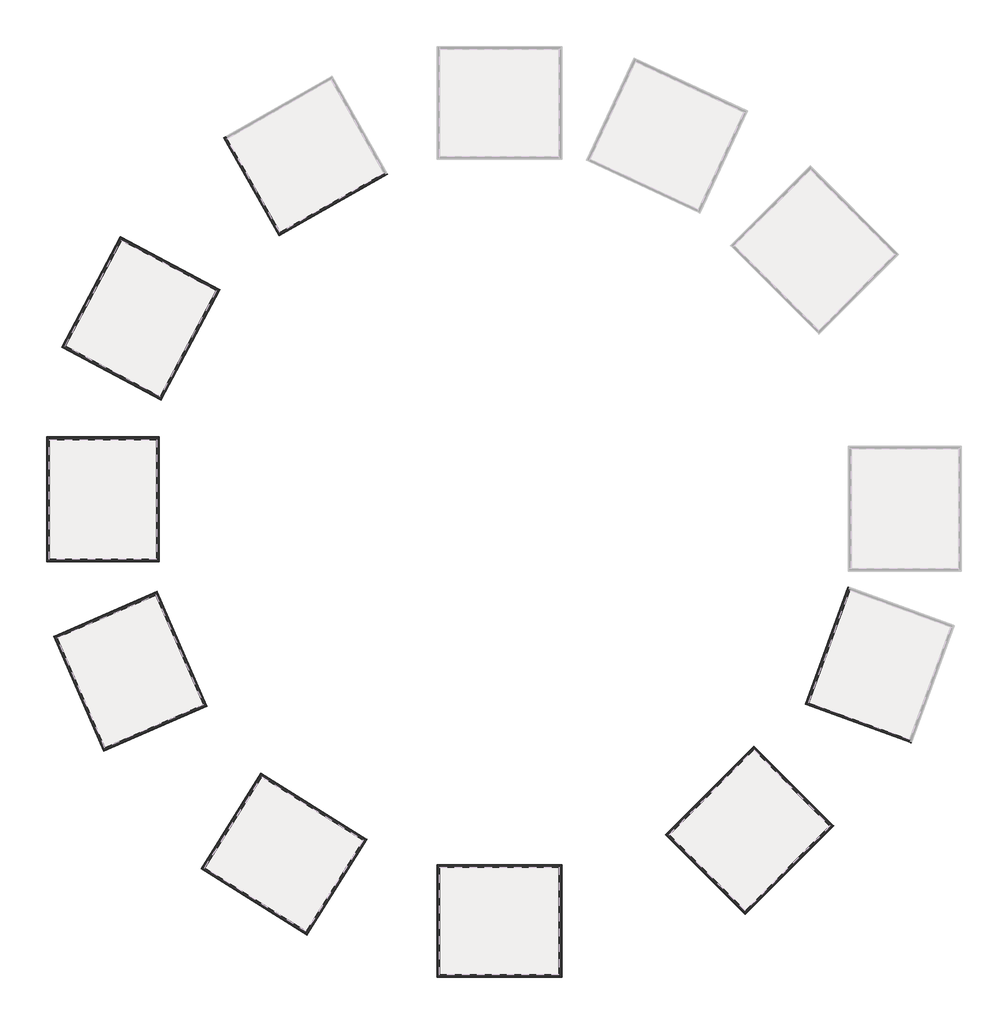
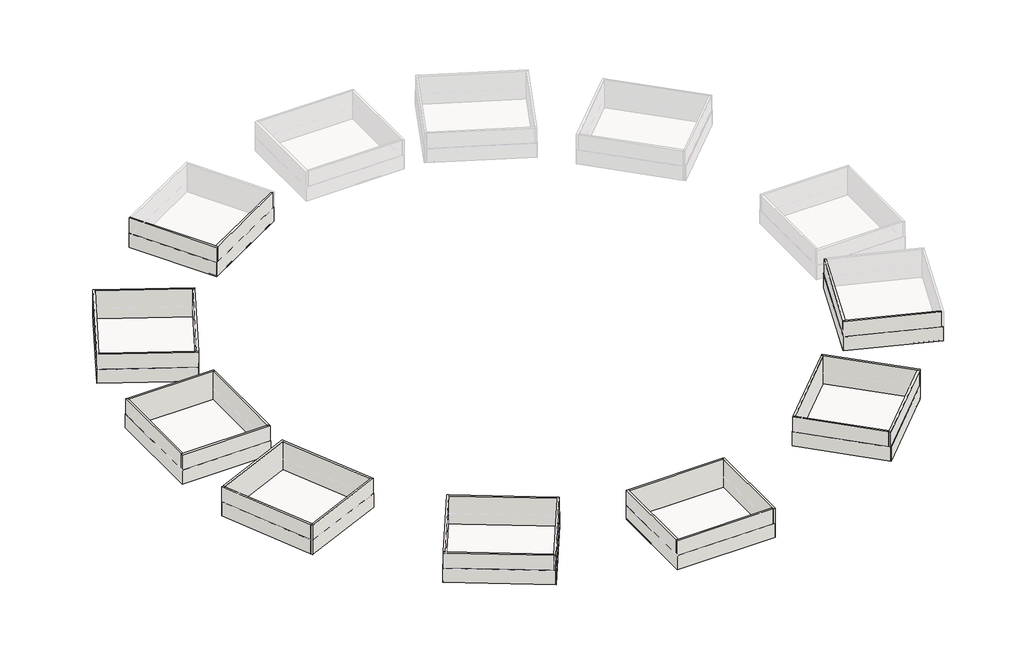
# One storey, part 1 of 2: 56 walls.
"""IFC4 building model written with IfcOpenShell, lengths in millimetres."""

from ifc_helpers import new_model, si_unit, origin, origin_with_axes, place, context, project, spatial, polyline, outline, extrude, faceted_brep, element, save

model = new_model("IFC4")

# Units and contexts
model_context = context("Model", 3, world=origin())
ifc_project = project(units=[si_unit("LENGTHUNIT", "METRE", prefix="MILLI")], contexts=[model_context])

# Site, building, storey
site = spatial("IfcSite", under=ifc_project)
building = spatial("IfcBuilding", under=site)
storey = spatial("IfcBuildingStorey", under=building, Name="01 этаж_+0.000", Elevation=0.0)

# Walls
placement = place(None, origin())
element("IfcWall", 1, ObjectType="Внутренняя_К380", at=placement, inside=storey, context=model_context, shape_type="Brep", body=[
    faceted_brep([(19810.0, -115810.0, 0.0), (19810.0, -116190.0, 0.0), (19810.0, -133810.0, 0.0), (19810.0, -134190.0, 0.0), (19810.0, -134190.0, 6380.0), (19810.0, -133810.0, 6380.0), (19810.0, -116190.0, 6380.0), (19810.0, -115810.0, 6380.0), (20190.0, -115810.0, 0.0), (20190.0, -115810.0, 6380.0), (20190.0, -134190.0, 6380.0), (20190.0, -134190.0, 0.0)], [[[0, 1, 2, 3, 4, 5, 6, 7]], [[8, 9, 10, 11]], [[3, 2, 1, 0, 8, 11]], [[7, 6, 5, 4, 10, 9]], [[4, 3, 11, 10]], [[0, 7, 9, 8]]]),
])
element("IfcWall", 2, ObjectType="Внутренняя_К380", at=placement, inside=storey, context=model_context, shape_type="Brep", body=[
    faceted_brep([(19810.0, -133810.0, 0.0), (190.0, -133810.0, 0.0), (-190.0, -133810.0, 0.0), (-190.0, -133810.0, 6380.0), (190.0, -133810.0, 6380.0), (19810.0, -133810.0, 6380.0), (19810.0, -134190.0, 0.0), (19810.0, -134190.0, 6380.0), (-190.0, -134190.0, 6380.0), (-190.0, -134190.0, 0.0)], [[[0, 1, 2, 3, 4, 5]], [[6, 7, 8, 9]], [[2, 1, 0, 6, 9]], [[5, 4, 3, 8, 7]], [[0, 5, 7, 6]], [[3, 2, 9, 8]]]),
])
element("IfcWall", 3, ObjectType="Внутренняя_К380", at=placement, inside=storey, context=model_context, shape_type="Brep", body=[
    faceted_brep([(190.0, -133810.0, 0.0), (190.0, -116190.0, 0.0), (190.0, -115810.0, 0.0), (190.0, -115810.0, 6380.0), (190.0, -116190.0, 6380.0), (190.0, -133810.0, 6380.0), (-190.0, -133810.0, 0.0), (-190.0, -133810.0, 6380.0), (-190.0, -115810.0, 6380.0), (-190.0, -115810.0, 0.0)], [[[0, 1, 2, 3, 4, 5]], [[6, 7, 8, 9]], [[2, 1, 0, 6, 9]], [[5, 4, 3, 8, 7]], [[0, 5, 7, 6]], [[3, 2, 9, 8]]]),
])
element("IfcWall", 4, ObjectType="Внутренняя_К380", at=placement, inside=storey, context=model_context, shape_type="SweptSolid", body=[
    extrude(outline(polyline([(19810.0, -116190.0), (190.0, -116190.0), (190.0, -115810.0), (19810.0, -115810.0), (19810.0, -116190.0)])), origin_with_axes(), (0.0, 0.0, 1.0), 6380.0),
])
element("IfcWall", 5, ObjectType="ОС-01 Окраска цвет белый 5мм", at=placement, inside=storey, context=model_context, shape_type="Brep", body=[
    faceted_brep([(20240.0, -134190.0, 0.0), (20190.0, -134190.0, 0.0), (-190.0, -134190.0, 0.0), (-240.0, -134190.0, 0.0), (-240.0, -134190.0, 3080.0), (-190.0, -134190.0, 3080.0), (20190.0, -134190.0, 3080.0), (20240.0, -134190.0, 3080.0), (20240.0, -134240.0, 0.0), (20240.0, -134240.0, 3080.0), (-240.0, -134240.0, 3080.0), (-240.0, -134240.0, 0.0)], [[[0, 1, 2, 3, 4, 5, 6, 7]], [[8, 9, 10, 11]], [[3, 2, 1, 0, 8, 11]], [[7, 6, 5, 4, 10, 9]], [[0, 7, 9, 8]], [[4, 3, 11, 10]]]),
])
element("IfcWall", 6, ObjectType="ОС-01 Окраска цвет белый 5мм", at=placement, inside=storey, context=model_context, shape_type="Brep", body=[
    faceted_brep([(20240.0, -134190.0, 0.0), (20240.0, -115760.0, 0.0), (20240.0, -115760.0, 3080.0), (20240.0, -134190.0, 3080.0), (20190.0, -134190.0, 0.0), (20190.0, -134190.0, 3080.0), (20190.0, -115810.0, 3080.0), (20190.0, -115760.0, 3080.0), (20190.0, -115760.0, 0.0), (20190.0, -115810.0, 0.0)], [[[0, 1, 2, 3]], [[4, 5, 6, 7, 8, 9]], [[1, 0, 4, 9, 8]], [[3, 2, 7, 6, 5]], [[0, 3, 5, 4]], [[2, 1, 8, 7]]]),
])
element("IfcWall", 7, ObjectType="ОС-01 Окраска цвет белый 5мм", at=placement, inside=storey, context=model_context, shape_type="Brep", body=[
    faceted_brep([(-190.0, -134190.0, 0.0), (-190.0, -115810.0, 0.0), (-190.0, -115760.0, 0.0), (-190.0, -115760.0, 3080.0), (-190.0, -115810.0, 3080.0), (-190.0, -134190.0, 3080.0), (-240.0, -134190.0, 0.0), (-240.0, -134190.0, 3080.0), (-240.0, -115760.0, 3080.0), (-240.0, -115760.0, 0.0)], [[[0, 1, 2, 3, 4, 5]], [[6, 7, 8, 9]], [[2, 1, 0, 6, 9]], [[5, 4, 3, 8, 7]], [[0, 5, 7, 6]], [[3, 2, 9, 8]]]),
])
element("IfcWall", 8, ObjectType="ОС-01 Окраска цвет белый 5мм", at=placement, inside=storey, context=model_context, shape_type="SweptSolid", body=[
    extrude(outline(polyline([(-190.0, -115760.0), (20190.0, -115760.0), (20190.0, -115810.0), (-190.0, -115810.0), (-190.0, -115760.0)])), origin_with_axes(), (0.0, 0.0, 1.0), 3080.0),
])
element("IfcWall", 9, ObjectType="Внутренняя_К380", at=placement, inside=storey, context=model_context, shape_type="Brep", body=[
    faceted_brep([(-45765.4225187, -65750.266627, 0.0), (-46145.4225187, -65750.266627, 0.0), (-63765.4225187, -65750.266627, 0.0), (-64145.4225187, -65750.266627, 0.0), (-64145.4225187, -65750.266627, 6380.0), (-63765.4225187, -65750.266627, 6380.0), (-46145.4225187, -65750.266627, 6380.0), (-45765.4225187, -65750.266627, 6380.0), (-45765.4225187, -66130.266627, 0.0), (-45765.4225187, -66130.266627, 6380.0), (-64145.4225187, -66130.266627, 6380.0), (-64145.4225187, -66130.266627, 0.0)], [[[0, 1, 2, 3, 4, 5, 6, 7]], [[8, 9, 10, 11]], [[3, 2, 1, 0, 8, 11]], [[7, 6, 5, 4, 10, 9]], [[4, 3, 11, 10]], [[0, 7, 9, 8]]]),
])
element("IfcWall", 10, ObjectType="Внутренняя_К380", at=placement, inside=storey, context=model_context, shape_type="Brep", body=[
    faceted_brep([(-63765.4225187, -65750.266627, 0.0), (-63765.4225187, -46130.266627, 0.0), (-63765.4225187, -45750.266627, 0.0), (-63765.4225187, -45750.266627, 6380.0), (-63765.4225187, -46130.266627, 6380.0), (-63765.4225187, -65750.266627, 6380.0), (-64145.4225187, -65750.266627, 0.0), (-64145.4225187, -65750.266627, 6380.0), (-64145.4225187, -45750.266627, 6380.0), (-64145.4225187, -45750.266627, 0.0)], [[[0, 1, 2, 3, 4, 5]], [[6, 7, 8, 9]], [[2, 1, 0, 6, 9]], [[5, 4, 3, 8, 7]], [[0, 5, 7, 6]], [[3, 2, 9, 8]]]),
])
element("IfcWall", 11, ObjectType="Внутренняя_К380", at=placement, inside=storey, context=model_context, shape_type="Brep", body=[
    faceted_brep([(-63765.4225187, -46130.266627, 0.0), (-46145.4225187, -46130.266627, 0.0), (-45765.4225187, -46130.266627, 0.0), (-45765.4225187, -46130.266627, 6380.0), (-46145.4225187, -46130.266627, 6380.0), (-63765.4225187, -46130.266627, 6380.0), (-63765.4225187, -45750.266627, 0.0), (-63765.4225187, -45750.266627, 6380.0), (-45765.4225187, -45750.266627, 6380.0), (-45765.4225187, -45750.266627, 0.0)], [[[0, 1, 2, 3, 4, 5]], [[6, 7, 8, 9]], [[2, 1, 0, 6, 9]], [[5, 4, 3, 8, 7]], [[0, 5, 7, 6]], [[3, 2, 9, 8]]]),
])
element("IfcWall", 12, ObjectType="Внутренняя_К380", at=placement, inside=storey, context=model_context, shape_type="SweptSolid", body=[
    extrude(outline(polyline([(-46145.4225187, -65750.266627), (-46145.4225187, -46130.266627), (-45765.4225187, -46130.266627), (-45765.4225187, -65750.266627), (-46145.4225187, -65750.266627)])), origin_with_axes(), (0.0, 0.0, 1.0), 6380.0),
])
element("IfcWall", 13, ObjectType="ОС-01 Окраска цвет белый 5мм", at=placement, inside=storey, context=model_context, shape_type="Brep", body=[
    faceted_brep([(-64145.4225187, -66180.266627, 0.0), (-64145.4225187, -66130.266627, 0.0), (-64145.4225187, -45750.266627, 0.0), (-64145.4225187, -45700.266627, 0.0), (-64145.4225187, -45700.266627, 3080.0), (-64145.4225187, -45750.266627, 3080.0), (-64145.4225187, -66130.266627, 3080.0), (-64145.4225187, -66180.266627, 3080.0), (-64195.4225187, -66180.266627, 0.0), (-64195.4225187, -66180.266627, 3080.0), (-64195.4225187, -45700.266627, 3080.0), (-64195.4225187, -45700.266627, 0.0)], [[[0, 1, 2, 3, 4, 5, 6, 7]], [[8, 9, 10, 11]], [[3, 2, 1, 0, 8, 11]], [[7, 6, 5, 4, 10, 9]], [[0, 7, 9, 8]], [[4, 3, 11, 10]]]),
])
element("IfcWall", 14, ObjectType="ОС-01 Окраска цвет белый 5мм", at=placement, inside=storey, context=model_context, shape_type="Brep", body=[
    faceted_brep([(-64145.4225187, -66180.266627, 0.0), (-45715.4225187, -66180.266627, 0.0), (-45715.4225187, -66180.266627, 3080.0), (-64145.4225187, -66180.266627, 3080.0), (-64145.4225187, -66130.266627, 0.0), (-64145.4225187, -66130.266627, 3080.0), (-45765.4225187, -66130.266627, 3080.0), (-45715.4225187, -66130.266627, 3080.0), (-45715.4225187, -66130.266627, 0.0), (-45765.4225187, -66130.266627, 0.0)], [[[0, 1, 2, 3]], [[4, 5, 6, 7, 8, 9]], [[1, 0, 4, 9, 8]], [[3, 2, 7, 6, 5]], [[0, 3, 5, 4]], [[2, 1, 8, 7]]]),
])
element("IfcWall", 15, ObjectType="ОС-01 Окраска цвет белый 5мм", at=placement, inside=storey, context=model_context, shape_type="Brep", body=[
    faceted_brep([(-64145.4225187, -45750.266627, 0.0), (-45765.4225187, -45750.266627, 0.0), (-45715.4225187, -45750.266627, 0.0), (-45715.4225187, -45750.266627, 3080.0), (-45765.4225187, -45750.266627, 3080.0), (-64145.4225187, -45750.266627, 3080.0), (-64145.4225187, -45700.266627, 0.0), (-64145.4225187, -45700.266627, 3080.0), (-45715.4225187, -45700.266627, 3080.0), (-45715.4225187, -45700.266627, 0.0)], [[[0, 1, 2, 3, 4, 5]], [[6, 7, 8, 9]], [[2, 1, 0, 6, 9]], [[5, 4, 3, 8, 7]], [[0, 5, 7, 6]], [[3, 2, 9, 8]]]),
])
element("IfcWall", 16, ObjectType="ОС-01 Окраска цвет белый 5мм", at=placement, inside=storey, context=model_context, shape_type="SweptSolid", body=[
    extrude(outline(polyline([(-45715.4225187, -45750.266627), (-45715.4225187, -66130.266627), (-45765.4225187, -66130.266627), (-45765.4225187, -45750.266627), (-45715.4225187, -45750.266627)])), origin_with_axes(), (0.0, 0.0, 1.0), 3080.0),
])
element("IfcWall", 17, ObjectType="Внутренняя_К380", at=placement, inside=storey, context=model_context, shape_type="Brep", body=[
    faceted_brep([(77278.5984613, -95287.4997432, 0.0), (60721.2144831, -89261.1048178, 0.0), (60364.1312872, -89131.1371634, 0.0), (60364.1312872, -89131.1371634, 6380.0), (60721.2144831, -89261.1048178, 6380.0), (77278.5984613, -95287.4997432, 6380.0), (77148.6308069, -95644.5829391, 0.0), (77148.6308069, -95644.5829391, 6380.0), (60234.1636327, -89488.2203593, 6380.0), (60234.1636327, -89488.2203593, 0.0)], [[[0, 1, 2, 3, 4, 5]], [[6, 7, 8, 9]], [[2, 1, 0, 6, 9]], [[5, 4, 3, 8, 7]], [[0, 5, 7, 6]], [[3, 2, 9, 8]]]),
])
element("IfcWall", 18, ObjectType="Внутренняя_К380", at=placement, inside=storey, context=model_context, shape_type="SweptSolid", body=[
    extrude(outline(polyline([(67431.6496951, -70824.335598), (60721.2144831, -89261.1048178), (60364.1312872, -89131.1371634), (67074.5664992, -70694.3679435), (67431.6496951, -70824.335598)])), origin_with_axes(), (0.0, 0.0, 1.0), 6380.0),
])
element("IfcWall", 19, ObjectType="ОС-01 Окраска цвет белый 5мм", at=placement, inside=storey, context=model_context, shape_type="Brep", body=[
    faceted_brep([(77505.7140028, -95774.5505936, 0.0), (60234.1636327, -89488.2203593, 0.0), (60187.1790017, -89471.1193521, 0.0), (60187.1790017, -89471.1193521, 3080.0), (60234.1636327, -89488.2203593, 3080.0), (77505.7140028, -95774.5505936, 3080.0), (77488.6129956, -95821.5352246, 0.0), (77488.6129956, -95821.5352246, 3080.0), (60170.0779945, -89518.1039831, 3080.0), (60170.0779945, -89518.1039831, 0.0)], [[[0, 1, 2, 3, 4, 5]], [[6, 7, 8, 9]], [[2, 1, 0, 6, 9]], [[5, 4, 3, 8, 7]], [[0, 5, 7, 6]], [[3, 2, 9, 8]]]),
])
element("IfcWall", 20, ObjectType="ОС-01 Окраска цвет белый 5мм", at=placement, inside=storey, context=model_context, shape_type="SweptSolid", body=[
    extrude(outline(polyline([(60187.1790017, -89471.1193521), (67157.5495227, -70320.1837405), (67204.5341537, -70337.2847476), (60234.1636327, -89488.2203593), (60187.1790017, -89471.1193521)])), origin_with_axes(), (0.0, 0.0, 1.0), 3080.0),
])
element("IfcWall", 21, ObjectType="Внутренняя_К380", at=placement, inside=storey, context=model_context, shape_type="Brep", body=[
    faceted_brep([(51459.9936659, -96700.311683, 0.0), (51728.6942428, -96969.0122598, 0.0), (64187.9157273, -109428.2337443, 0.0), (64456.6163041, -109696.9343212, 0.0), (64456.6163041, -109696.9343212, 6380.0), (64187.9157273, -109428.2337443, 6380.0), (51728.6942428, -96969.0122598, 6380.0), (51459.9936659, -96700.311683, 6380.0), (51728.6942428, -96431.6111061, 0.0), (51728.6942428, -96431.6111061, 6380.0), (64725.316881, -109428.2337443, 6380.0), (64725.316881, -109428.2337443, 0.0)], [[[0, 1, 2, 3, 4, 5, 6, 7]], [[8, 9, 10, 11]], [[3, 2, 1, 0, 8, 11]], [[7, 6, 5, 4, 10, 9]], [[4, 3, 11, 10]], [[0, 7, 9, 8]]]),
])
element("IfcWall", 22, ObjectType="Внутренняя_К380", at=placement, inside=storey, context=model_context, shape_type="Brep", body=[
    faceted_brep([(64187.9157273, -109428.2337443, 0.0), (50314.4806804, -123301.6687912, 0.0), (50045.7801036, -123570.3693681, 0.0), (50045.7801036, -123570.3693681, 6380.0), (50314.4806804, -123301.6687912, 6380.0), (64187.9157273, -109428.2337443, 6380.0), (64456.6163041, -109696.9343212, 0.0), (64456.6163041, -109696.9343212, 6380.0), (50314.4806804, -123839.0699449, 6380.0), (50314.4806804, -123839.0699449, 0.0)], [[[0, 1, 2, 3, 4, 5]], [[6, 7, 8, 9]], [[2, 1, 0, 6, 9]], [[5, 4, 3, 8, 7]], [[0, 5, 7, 6]], [[3, 2, 9, 8]]]),
])
element("IfcWall", 23, ObjectType="Внутренняя_К380", at=placement, inside=storey, context=model_context, shape_type="Brep", body=[
    faceted_brep([(50314.4806804, -123301.6687912, 0.0), (37855.2591959, -110842.4473067, 0.0), (37586.5586191, -110573.7467298, 0.0), (37586.5586191, -110573.7467298, 6380.0), (37855.2591959, -110842.4473067, 6380.0), (50314.4806804, -123301.6687912, 6380.0), (50045.7801036, -123570.3693681, 0.0), (50045.7801036, -123570.3693681, 6380.0), (37317.8580422, -110842.4473067, 6380.0), (37317.8580422, -110842.4473067, 0.0)], [[[0, 1, 2, 3, 4, 5]], [[6, 7, 8, 9]], [[2, 1, 0, 6, 9]], [[5, 4, 3, 8, 7]], [[0, 5, 7, 6]], [[3, 2, 9, 8]]]),
])
element("IfcWall", 24, ObjectType="Внутренняя_К380", at=placement, inside=storey, context=model_context, shape_type="SweptSolid", body=[
    extrude(outline(polyline([(51728.6942428, -96969.0122598), (37855.2591959, -110842.4473067), (37586.5586191, -110573.7467298), (51459.9936659, -96700.311683), (51728.6942428, -96969.0122598)])), origin_with_axes(), (0.0, 0.0, 1.0), 6380.0),
])
element("IfcWall", 25, ObjectType="ОС-01 Окраска цвет белый 5мм", at=placement, inside=storey, context=model_context, shape_type="Brep", body=[
    faceted_brep([(64760.6722201, -109392.8784053, 0.0), (64725.316881, -109428.2337443, 0.0), (50314.4806804, -123839.0699449, 0.0), (50279.1253414, -123874.425284, 0.0), (50279.1253414, -123874.425284, 3080.0), (50314.4806804, -123839.0699449, 3080.0), (64725.316881, -109428.2337443, 3080.0), (64760.6722201, -109392.8784053, 3080.0), (64796.0275591, -109428.2337443, 0.0), (64796.0275591, -109428.2337443, 3080.0), (50314.4806804, -123909.780623, 3080.0), (50314.4806804, -123909.780623, 0.0)], [[[0, 1, 2, 3, 4, 5, 6, 7]], [[8, 9, 10, 11]], [[3, 2, 1, 0, 8, 11]], [[7, 6, 5, 4, 10, 9]], [[0, 7, 9, 8]], [[4, 3, 11, 10]]]),
])
element("IfcWall", 26, ObjectType="ОС-01 Окраска цвет белый 5мм", at=placement, inside=storey, context=model_context, shape_type="Brep", body=[
    faceted_brep([(64760.6722201, -109392.8784053, 0.0), (51728.6942428, -96360.900428, 0.0), (51728.6942428, -96360.900428, 3080.0), (64760.6722201, -109392.8784053, 3080.0), (64725.316881, -109428.2337443, 0.0), (64725.316881, -109428.2337443, 3080.0), (51728.6942428, -96431.6111061, 3080.0), (51693.3389037, -96396.2557671, 3080.0), (51693.3389037, -96396.2557671, 0.0), (51728.6942428, -96431.6111061, 0.0)], [[[0, 1, 2, 3]], [[4, 5, 6, 7, 8, 9]], [[1, 0, 4, 9, 8]], [[3, 2, 7, 6, 5]], [[0, 3, 5, 4]], [[2, 1, 8, 7]]]),
])
element("IfcWall", 27, ObjectType="ОС-01 Окраска цвет белый 5мм", at=placement, inside=storey, context=model_context, shape_type="Brep", body=[
    faceted_brep([(50314.4806804, -123839.0699449, 0.0), (37317.8580422, -110842.4473067, 0.0), (37282.5027031, -110807.0919676, 0.0), (37282.5027031, -110807.0919676, 3080.0), (37317.8580422, -110842.4473067, 3080.0), (50314.4806804, -123839.0699449, 3080.0), (50279.1253414, -123874.425284, 0.0), (50279.1253414, -123874.425284, 3080.0), (37247.1473641, -110842.4473067, 3080.0), (37247.1473641, -110842.4473067, 0.0)], [[[0, 1, 2, 3, 4, 5]], [[6, 7, 8, 9]], [[2, 1, 0, 6, 9]], [[5, 4, 3, 8, 7]], [[0, 5, 7, 6]], [[3, 2, 9, 8]]]),
])
element("IfcWall", 28, ObjectType="ОС-01 Окраска цвет белый 5мм", at=placement, inside=storey, context=model_context, shape_type="SweptSolid", body=[
    extrude(outline(polyline([(37282.5027031, -110807.0919676), (51693.3389037, -96396.2557671), (51728.6942428, -96431.6111061), (37317.8580422, -110842.4473067), (37282.5027031, -110807.0919676)])), origin_with_axes(), (0.0, 0.0, 1.0), 3080.0),
])
element("IfcWall", 29, ObjectType="Внутренняя_К380", at=placement, inside=storey, context=model_context, shape_type="Brep", body=[
    faceted_brep([(-12092.271683, -111446.4430586, 0.0), (-12293.6410034, -111768.7013351, 0.0), (-21630.8184392, -126711.3087894, 0.0), (-21832.1877596, -127033.5670659, 0.0), (-21832.1877596, -127033.5670659, 6380.0), (-21630.8184392, -126711.3087894, 6380.0), (-12293.6410034, -111768.7013351, 6380.0), (-12092.271683, -111446.4430586, 6380.0), (-11770.0134064, -111647.812379, 0.0), (-11770.0134064, -111647.812379, 6380.0), (-21509.929483, -127234.9363863, 6380.0), (-21509.929483, -127234.9363863, 0.0)], [[[0, 1, 2, 3, 4, 5, 6, 7]], [[8, 9, 10, 11]], [[3, 2, 1, 0, 8, 11]], [[7, 6, 5, 4, 10, 9]], [[4, 3, 11, 10]], [[0, 7, 9, 8]]]),
])
element("IfcWall", 30, ObjectType="Внутренняя_К380", at=placement, inside=storey, context=model_context, shape_type="Brep", body=[
    faceted_brep([(-21630.8184392, -126711.3087894, 0.0), (-38269.5220858, -116314.2928251, 0.0), (-38591.7803623, -116112.9235047, 0.0), (-38591.7803623, -116112.9235047, 6380.0), (-38269.5220858, -116314.2928251, 6380.0), (-21630.8184392, -126711.3087894, 6380.0), (-21832.1877596, -127033.5670659, 0.0), (-21832.1877596, -127033.5670659, 6380.0), (-38793.1496827, -116435.1817812, 6380.0), (-38793.1496827, -116435.1817812, 0.0)], [[[0, 1, 2, 3, 4, 5]], [[6, 7, 8, 9]], [[2, 1, 0, 6, 9]], [[5, 4, 3, 8, 7]], [[0, 5, 7, 6]], [[3, 2, 9, 8]]]),
])
element("IfcWall", 31, ObjectType="Внутренняя_К380", at=placement, inside=storey, context=model_context, shape_type="Brep", body=[
    faceted_brep([(-38269.5220858, -116314.2928251, 0.0), (-28932.34465, -101371.6853708, 0.0), (-28730.9753296, -101049.4270943, 0.0), (-28730.9753296, -101049.4270943, 6380.0), (-28932.34465, -101371.6853708, 6380.0), (-38269.5220858, -116314.2928251, 6380.0), (-38591.7803623, -116112.9235047, 0.0), (-38591.7803623, -116112.9235047, 6380.0), (-29053.2336061, -100848.0577739, 6380.0), (-29053.2336061, -100848.0577739, 0.0)], [[[0, 1, 2, 3, 4, 5]], [[6, 7, 8, 9]], [[2, 1, 0, 6, 9]], [[5, 4, 3, 8, 7]], [[0, 5, 7, 6]], [[3, 2, 9, 8]]]),
])
element("IfcWall", 32, ObjectType="Внутренняя_К380", at=placement, inside=storey, context=model_context, shape_type="SweptSolid", body=[
    extrude(outline(polyline([(-12293.6410034, -111768.7013351), (-28932.34465, -101371.6853708), (-28730.9753296, -101049.4270943), (-12092.271683, -111446.4430586), (-12293.6410034, -111768.7013351)])), origin_with_axes(), (0.0, 0.0, 1.0), 6380.0),
])
element("IfcWall", 33, ObjectType="ОС-01 Окраска цвет белый 5мм", at=placement, inside=storey, context=model_context, shape_type="Brep", body=[
    faceted_brep([(-21467.5270782, -127261.4323495, 0.0), (-21509.929483, -127234.9363863, 0.0), (-38793.1496827, -116435.1817812, 0.0), (-38835.5520875, -116408.685818, 0.0), (-38835.5520875, -116408.685818, 3080.0), (-38793.1496827, -116435.1817812, 3080.0), (-21509.929483, -127234.9363863, 3080.0), (-21467.5270782, -127261.4323495, 3080.0), (-21494.0230414, -127303.8347543, 0.0), (-21494.0230414, -127303.8347543, 3080.0), (-38862.0480507, -116451.0882228, 3080.0), (-38862.0480507, -116451.0882228, 0.0)], [[[0, 1, 2, 3, 4, 5, 6, 7]], [[8, 9, 10, 11]], [[3, 2, 1, 0, 8, 11]], [[7, 6, 5, 4, 10, 9]], [[0, 7, 9, 8]], [[4, 3, 11, 10]]]),
])
element("IfcWall", 34, ObjectType="ОС-01 Окраска цвет белый 5мм", at=placement, inside=storey, context=model_context, shape_type="Brep", body=[
    faceted_brep([(-21467.5270782, -127261.4323495, 0.0), (-11701.1150384, -111631.9059374, 0.0), (-11701.1150384, -111631.9059374, 3080.0), (-21467.5270782, -127261.4323495, 3080.0), (-21509.929483, -127234.9363863, 0.0), (-21509.929483, -127234.9363863, 3080.0), (-11770.0134064, -111647.812379, 3080.0), (-11743.5174432, -111605.4099742, 3080.0), (-11743.5174432, -111605.4099742, 0.0), (-11770.0134064, -111647.812379, 0.0)], [[[0, 1, 2, 3]], [[4, 5, 6, 7, 8, 9]], [[1, 0, 4, 9, 8]], [[3, 2, 7, 6, 5]], [[0, 3, 5, 4]], [[2, 1, 8, 7]]]),
])
element("IfcWall", 35, ObjectType="ОС-01 Окраска цвет белый 5мм", at=placement, inside=storey, context=model_context, shape_type="Brep", body=[
    faceted_brep([(-38793.1496827, -116435.1817812, 0.0), (-29053.2336061, -100848.0577739, 0.0), (-29026.7376429, -100805.6553691, 0.0), (-29026.7376429, -100805.6553691, 3080.0), (-29053.2336061, -100848.0577739, 3080.0), (-38793.1496827, -116435.1817812, 3080.0), (-38835.5520875, -116408.685818, 0.0), (-38835.5520875, -116408.685818, 3080.0), (-29069.1400477, -100779.1594059, 3080.0), (-29069.1400477, -100779.1594059, 0.0)], [[[0, 1, 2, 3, 4, 5]], [[6, 7, 8, 9]], [[2, 1, 0, 6, 9]], [[5, 4, 3, 8, 7]], [[0, 5, 7, 6]], [[3, 2, 9, 8]]]),
])
element("IfcWall", 36, ObjectType="ОС-01 Окраска цвет белый 5мм", at=placement, inside=storey, context=model_context, shape_type="SweptSolid", body=[
    extrude(outline(polyline([(-29026.7376429, -100805.6553691), (-11743.5174432, -111605.4099742), (-11770.0134064, -111647.812379), (-29053.2336061, -100848.0577739), (-29026.7376429, -100805.6553691)])), origin_with_axes(), (0.0, 0.0, 1.0), 3080.0),
])
element("IfcWall", 37, ObjectType="Внутренняя_К380", at=placement, inside=storey, context=model_context, shape_type="Brep", body=[
    faceted_brep([(-38115.4224369, -89424.2884282, 0.0), (-38463.9052652, -89575.8130744, 0.0), (-54622.5037758, -96601.7716689, 0.0), (-54970.9866041, -96753.2963151, 0.0), (-54970.9866041, -96753.2963151, 6380.0), (-54622.5037758, -96601.7716689, 6380.0), (-38463.9052652, -89575.8130744, 6380.0), (-38115.4224369, -89424.2884282, 6380.0), (-37963.8977907, -89772.7712565, 0.0), (-37963.8977907, -89772.7712565, 6380.0), (-54819.4619579, -97101.7791433, 6380.0), (-54819.4619579, -97101.7791433, 0.0)], [[[0, 1, 2, 3, 4, 5, 6, 7]], [[8, 9, 10, 11]], [[3, 2, 1, 0, 8, 11]], [[7, 6, 5, 4, 10, 9]], [[4, 3, 11, 10]], [[0, 7, 9, 8]]]),
])
element("IfcWall", 38, ObjectType="Внутренняя_К380", at=placement, inside=storey, context=model_context, shape_type="Brep", body=[
    faceted_brep([(-54622.5037758, -96601.7716689, 0.0), (-62445.9605082, -78609.0530095, 0.0), (-62597.4851543, -78260.5701812, 0.0), (-62597.4851543, -78260.5701812, 6380.0), (-62445.9605082, -78609.0530095, 6380.0), (-54622.5037758, -96601.7716689, 6380.0), (-54970.9866041, -96753.2963151, 0.0), (-54970.9866041, -96753.2963151, 6380.0), (-62945.9679826, -78412.0948274, 6380.0), (-62945.9679826, -78412.0948274, 0.0)], [[[0, 1, 2, 3, 4, 5]], [[6, 7, 8, 9]], [[2, 1, 0, 6, 9]], [[5, 4, 3, 8, 7]], [[0, 5, 7, 6]], [[3, 2, 9, 8]]]),
])
element("IfcWall", 39, ObjectType="Внутренняя_К380", at=placement, inside=storey, context=model_context, shape_type="Brep", body=[
    faceted_brep([(-62445.9605082, -78609.0530095, 0.0), (-46287.3619975, -71583.094415, 0.0), (-45938.8791692, -71431.5697688, 0.0), (-45938.8791692, -71431.5697688, 6380.0), (-46287.3619975, -71583.094415, 6380.0), (-62445.9605082, -78609.0530095, 6380.0), (-62597.4851543, -78260.5701812, 0.0), (-62597.4851543, -78260.5701812, 6380.0), (-46090.4038154, -71083.0869405, 6380.0), (-46090.4038154, -71083.0869405, 0.0)], [[[0, 1, 2, 3, 4, 5]], [[6, 7, 8, 9]], [[2, 1, 0, 6, 9]], [[5, 4, 3, 8, 7]], [[0, 5, 7, 6]], [[3, 2, 9, 8]]]),
])
element("IfcWall", 40, ObjectType="Внутренняя_К380", at=placement, inside=storey, context=model_context, shape_type="SweptSolid", body=[
    extrude(outline(polyline([(-38463.9052652, -89575.8130744), (-46287.3619975, -71583.094415), (-45938.8791692, -71431.5697688), (-38115.4224369, -89424.2884282), (-38463.9052652, -89575.8130744)])), origin_with_axes(), (0.0, 0.0, 1.0), 6380.0),
])
element("IfcWall", 41, ObjectType="ОС-01 Окраска цвет белый 5мм", at=placement, inside=storey, context=model_context, shape_type="Brep", body=[
    faceted_brep([(-54799.5245045, -97147.6321471, 0.0), (-54819.4619579, -97101.7791433, 0.0), (-62945.9679826, -78412.0948274, 0.0), (-62965.9054361, -78366.2418237, 0.0), (-62965.9054361, -78366.2418237, 3080.0), (-62945.9679826, -78412.0948274, 3080.0), (-54819.4619579, -97101.7791433, 3080.0), (-54799.5245045, -97147.6321471, 3080.0), (-54845.3775082, -97167.5696005, 0.0), (-54845.3775082, -97167.5696005, 3080.0), (-63011.7584398, -78386.1792771, 3080.0), (-63011.7584398, -78386.1792771, 0.0)], [[[0, 1, 2, 3, 4, 5, 6, 7]], [[8, 9, 10, 11]], [[3, 2, 1, 0, 8, 11]], [[7, 6, 5, 4, 10, 9]], [[0, 7, 9, 8]], [[4, 3, 11, 10]]]),
])
element("IfcWall", 42, ObjectType="ОС-01 Окраска цвет белый 5мм", at=placement, inside=storey, context=model_context, shape_type="Brep", body=[
    faceted_brep([(-54799.5245045, -97147.6321471, 0.0), (-37898.1073336, -89798.6868068, 0.0), (-37898.1073336, -89798.6868068, 3080.0), (-54799.5245045, -97147.6321471, 3080.0), (-54819.4619579, -97101.7791433, 0.0), (-54819.4619579, -97101.7791433, 3080.0), (-37963.8977907, -89772.7712565, 3080.0), (-37918.044787, -89752.8338031, 3080.0), (-37918.044787, -89752.8338031, 0.0), (-37963.8977907, -89772.7712565, 0.0)], [[[0, 1, 2, 3]], [[4, 5, 6, 7, 8, 9]], [[1, 0, 4, 9, 8]], [[3, 2, 7, 6, 5]], [[0, 3, 5, 4]], [[2, 1, 8, 7]]]),
])
element("IfcWall", 43, ObjectType="ОС-01 Окраска цвет белый 5мм", at=placement, inside=storey, context=model_context, shape_type="Brep", body=[
    faceted_brep([(-62945.9679826, -78412.0948274, 0.0), (-46090.4038154, -71083.0869405, 0.0), (-46044.5508117, -71063.1494871, 0.0), (-46044.5508117, -71063.1494871, 3080.0), (-46090.4038154, -71083.0869405, 3080.0), (-62945.9679826, -78412.0948274, 3080.0), (-62965.9054361, -78366.2418237, 0.0), (-62965.9054361, -78366.2418237, 3080.0), (-46064.4882651, -71017.2964834, 3080.0), (-46064.4882651, -71017.2964834, 0.0)], [[[0, 1, 2, 3, 4, 5]], [[6, 7, 8, 9]], [[2, 1, 0, 6, 9]], [[5, 4, 3, 8, 7]], [[0, 5, 7, 6]], [[3, 2, 9, 8]]]),
])
element("IfcWall", 44, ObjectType="ОС-01 Окраска цвет белый 5мм", at=placement, inside=storey, context=model_context, shape_type="SweptSolid", body=[
    extrude(outline(polyline([(-46044.5508117, -71063.1494871), (-37918.044787, -89752.8338031), (-37963.8977907, -89772.7712565), (-46090.4038154, -71083.0869405), (-46044.5508117, -71063.1494871)])), origin_with_axes(), (0.0, 0.0, 1.0), 3080.0),
])
element("IfcWall", 45, ObjectType="Внутренняя_К380", at=placement, inside=storey, context=model_context, shape_type="Brep", body=[
    faceted_brep([(-45237.2003893, -39274.3010919, 0.0), (-45572.7204746, -39095.9018981, 0.0), (-61130.2570608, -30823.8129618, 0.0), (-61465.777146, -30645.4137679, 0.0), (-61465.777146, -30645.4137679, 6380.0), (-61130.2570608, -30823.8129618, 6380.0), (-45572.7204746, -39095.9018981, 6380.0), (-45237.2003893, -39274.3010919, 6380.0), (-45415.5995832, -39609.8211772, 0.0), (-45415.5995832, -39609.8211772, 6380.0), (-61644.1763399, -30980.9338532, 6380.0), (-61644.1763399, -30980.9338532, 0.0)], [[[0, 1, 2, 3, 4, 5, 6, 7]], [[8, 9, 10, 11]], [[3, 2, 1, 0, 8, 11]], [[7, 6, 5, 4, 10, 9]], [[4, 3, 11, 10]], [[0, 7, 9, 8]]]),
])
element("IfcWall", 46, ObjectType="Внутренняя_К380", at=placement, inside=storey, context=model_context, shape_type="Brep", body=[
    faceted_brep([(-61130.2570608, -30823.8129618, 0.0), (-51919.2249989, -13500.3811899, 0.0), (-51740.825805, -13164.8611046, 0.0), (-51740.825805, -13164.8611046, 6380.0), (-51919.2249989, -13500.3811899, 6380.0), (-61130.2570608, -30823.8129618, 6380.0), (-61465.777146, -30645.4137679, 0.0), (-61465.777146, -30645.4137679, 6380.0), (-52076.3458903, -12986.4619107, 6380.0), (-52076.3458903, -12986.4619107, 0.0)], [[[0, 1, 2, 3, 4, 5]], [[6, 7, 8, 9]], [[2, 1, 0, 6, 9]], [[5, 4, 3, 8, 7]], [[0, 5, 7, 6]], [[3, 2, 9, 8]]]),
])
element("IfcWall", 47, ObjectType="Внутренняя_К380", at=placement, inside=storey, context=model_context, shape_type="Brep", body=[
    faceted_brep([(-51919.2249989, -13500.3811899, 0.0), (-36361.6884127, -21772.4701262, 0.0), (-36026.1683274, -21950.86932, 0.0), (-36026.1683274, -21950.86932, 6380.0), (-36361.6884127, -21772.4701262, 6380.0), (-51919.2249989, -13500.3811899, 6380.0), (-51740.825805, -13164.8611046, 0.0), (-51740.825805, -13164.8611046, 6380.0), (-35847.7691336, -21615.3492347, 6380.0), (-35847.7691336, -21615.3492347, 0.0)], [[[0, 1, 2, 3, 4, 5]], [[6, 7, 8, 9]], [[2, 1, 0, 6, 9]], [[5, 4, 3, 8, 7]], [[0, 5, 7, 6]], [[3, 2, 9, 8]]]),
])
element("IfcWall", 48, ObjectType="Внутренняя_К380", at=placement, inside=storey, context=model_context, shape_type="SweptSolid", body=[
    extrude(outline(polyline([(-45572.7204746, -39095.9018981), (-36361.6884127, -21772.4701262), (-36026.1683274, -21950.86932), (-45237.2003893, -39274.3010919), (-45572.7204746, -39095.9018981)])), origin_with_axes(), (0.0, 0.0, 1.0), 6380.0),
])
element("IfcWall", 49, ObjectType="ОС-01 Окраска цвет белый 5мм", at=placement, inside=storey, context=model_context, shape_type="Brep", body=[
    faceted_brep([(-61667.649918, -31025.0812329, 0.0), (-61644.1763399, -30980.9338532, 0.0), (-52076.3458903, -12986.4619107, 0.0), (-52052.8723122, -12942.3145311, 0.0), (-52052.8723122, -12942.3145311, 3080.0), (-52076.3458903, -12986.4619107, 3080.0), (-61644.1763399, -30980.9338532, 3080.0), (-61667.649918, -31025.0812329, 3080.0), (-61711.7972977, -31001.6076547, 0.0), (-61711.7972977, -31001.6076547, 3080.0), (-52097.0196918, -12918.840953, 3080.0), (-52097.0196918, -12918.840953, 0.0)], [[[0, 1, 2, 3, 4, 5, 6, 7]], [[8, 9, 10, 11]], [[3, 2, 1, 0, 8, 11]], [[7, 6, 5, 4, 10, 9]], [[0, 7, 9, 8]], [[4, 3, 11, 10]]]),
])
element("IfcWall", 50, ObjectType="ОС-01 Окраска цвет белый 5мм", at=placement, inside=storey, context=model_context, shape_type="Brep", body=[
    faceted_brep([(-61667.649918, -31025.0812329, 0.0), (-45394.9257817, -39677.442135, 0.0), (-45394.9257817, -39677.442135, 3080.0), (-61667.649918, -31025.0812329, 3080.0), (-61644.1763399, -30980.9338532, 0.0), (-61644.1763399, -30980.9338532, 3080.0), (-45415.5995832, -39609.8211772, 3080.0), (-45371.4522035, -39633.2947554, 3080.0), (-45371.4522035, -39633.2947554, 0.0), (-45415.5995832, -39609.8211772, 0.0)], [[[0, 1, 2, 3]], [[4, 5, 6, 7, 8, 9]], [[1, 0, 4, 9, 8]], [[3, 2, 7, 6, 5]], [[0, 3, 5, 4]], [[2, 1, 8, 7]]]),
])
element("IfcWall", 51, ObjectType="ОС-01 Окраска цвет белый 5мм", at=placement, inside=storey, context=model_context, shape_type="Brep", body=[
    faceted_brep([(-52076.3458903, -12986.4619107, 0.0), (-35847.7691336, -21615.3492347, 0.0), (-35803.6217539, -21638.8228129, 0.0), (-35803.6217539, -21638.8228129, 3080.0), (-35847.7691336, -21615.3492347, 3080.0), (-52076.3458903, -12986.4619107, 3080.0), (-52052.8723122, -12942.3145311, 0.0), (-52052.8723122, -12942.3145311, 3080.0), (-35780.1481758, -21594.6754332, 3080.0), (-35780.1481758, -21594.6754332, 0.0)], [[[0, 1, 2, 3, 4, 5]], [[6, 7, 8, 9]], [[2, 1, 0, 6, 9]], [[5, 4, 3, 8, 7]], [[0, 5, 7, 6]], [[3, 2, 9, 8]]]),
])
element("IfcWall", 52, ObjectType="ОС-01 Окраска цвет белый 5мм", at=placement, inside=storey, context=model_context, shape_type="SweptSolid", body=[
    extrude(outline(polyline([(-35803.6217539, -21638.8228129), (-45371.4522035, -39633.2947554), (-45415.5995832, -39609.8211772), (-35847.7691336, -21615.3492347), (-35803.6217539, -21638.8228129)])), origin_with_axes(), (0.0, 0.0, 1.0), 3080.0),
])
element("IfcWall", 53, ObjectType="Внутренняя_К380", at=placement, inside=storey, context=model_context, shape_type="Brep", body=[
    faceted_brep([(-25758.700635, -12502.6801372, 0.0), (-25945.8215879, -12171.9449727, 0.0), (-34622.3247169, 3163.7223897, 0.0), (-34809.4456697, 3494.4575542, 0.0), (-34809.4456697, 3494.4575542, 6380.0), (-34622.3247169, 3163.7223897, 6380.0), (-25945.8215879, -12171.9449727, 6380.0), (-25758.700635, -12502.6801372, 6380.0), (-26089.4357995, -12689.80109, 0.0), (-26089.4357995, -12689.80109, 6380.0), (-35140.1808342, 3307.3366013, 6380.0), (-35140.1808342, 3307.3366013, 0.0)], [[[0, 1, 2, 3, 4, 5, 6, 7]], [[8, 9, 10, 11]], [[3, 2, 1, 0, 8, 11]], [[7, 6, 5, 4, 10, 9]], [[4, 3, 11, 10]], [[0, 7, 9, 8]]]),
])
element("IfcWall", 54, ObjectType="Внутренняя_К380", at=placement, inside=storey, context=model_context, shape_type="SweptSolid", body=[
    extrude(outline(polyline([(-25945.8215879, -12171.9449727), (-8869.4428335, -2510.5947235), (-8682.3218807, -2841.329888), (-25758.700635, -12502.6801372), (-25945.8215879, -12171.9449727)])), origin_with_axes(), (0.0, 0.0, 1.0), 6380.0),
])
element("IfcWall", 55, ObjectType="ОС-01 Окраска цвет белый 5мм", at=placement, inside=storey, context=model_context, shape_type="Brep", body=[
    faceted_brep([(-35183.698619, 3282.7154233, 0.0), (-26108.3324063, -12757.9400528, 0.0), (-26108.3324063, -12757.9400528, 3080.0), (-35183.698619, 3282.7154233, 3080.0), (-35140.1808342, 3307.3366013, 0.0), (-35140.1808342, 3307.3366013, 3080.0), (-26089.4357995, -12689.80109, 3080.0), (-26064.8146215, -12733.3188748, 3080.0), (-26064.8146215, -12733.3188748, 0.0), (-26089.4357995, -12689.80109, 0.0)], [[[0, 1, 2, 3]], [[4, 5, 6, 7, 8, 9]], [[1, 0, 4, 9, 8]], [[3, 2, 7, 6, 5]], [[0, 3, 5, 4]], [[2, 1, 8, 7]]]),
])
element("IfcWall", 56, ObjectType="ОС-01 Окраска цвет белый 5мм", at=placement, inside=storey, context=model_context, shape_type="SweptSolid", body=[
    extrude(outline(polyline([(-8326.9655382, -2697.7267199), (-26064.8146215, -12733.3188748), (-26089.4357995, -12689.80109), (-8351.5867162, -2654.2089351), (-8326.9655382, -2697.7267199)])), origin_with_axes(), (0.0, 0.0, 1.0), 3080.0),
])

save(model, "model.ifc")

# Revit data of these elements
# Project information
#   Название организации = "Название организации"
#   Наименование здания = "Введите наименование здания"
#   Разработчики шаблона = "Мехонцев Андрей Александрович"
#   Дата утверждения проекта = "1"
#   Статус проекта = "Р"
#   Заказчик = "Параметр не используется"
#   SR Document GUID = "c7b3c5ec-7626-4389-83ca-e13299f85324"
# Grids (mm)
#   "1": line (0, 20000) -> (0, -5134.966)
#   "А": line (20000, 0) -> (-5000, 0)
# Type "Внутренняя_К380"
#   Type Mark = "рап"
#   Layers, outside or top first: 380 mm "Кирпич керамический полтнотелый(штриховка 1:50)" (function 1)
# Type "ОС-01 Окраска цвет белый 5мм"
#   Model = "Отделка стен"
#   Type Mark = "ОС-01"
#   Layers, outside or top first: 50 mm "ОС-01 Окраска цвет белый" (function 5)
# Elements 1, 2, 3, 4, 9, 10, 11, 12, 17, 18, 21, 22, 23, 24, 29, 30, 31, 32, 37, 38, 39, 40, 45, 46, 47, 48, 53, 54 (IfcWall, "Внутренняя_К380")
#   Top Offset = -220 mm
#   Base Offset = 0 mm
#   wall height = 6380 mm
#   Phase Created = 1
#   Base Constraint = 01 этаж_+0.000
#   Top Constraint = 03 этаж_+6.600
#   Materials on its faces: "Кирпич керамический полтнотелый(штриховка 1:50)"
# Elements 5, 6, 7, 8, 13, 14, 15, 16, 19, 20, 25, 26, 27, 28, 33, 34, 35, 36, 41, 42, 43, 44, 49, 50, 51, 52, 55, 56 (IfcWall, "ОС-01 Окраска цвет белый 5мм")
#   Top Offset = -220 mm
#   Base Offset = 0 mm
#   wall height = 3080 mm
#   Phase Created = 1
#   Base Constraint = 01 этаж_+0.000
#   Top Constraint = 02 этаж_+3.300
#   Materials on its faces: "ОС-01 Окраска цвет белый"
# Materials
#   "Кирпич керамический полтнотелый(штриховка 1:50)": class "М150", colour RGB 170 100 105, transparency 0, Manufacturer = "Альтек", Description = "Керамический кирпич", Cost = 0
#   "ОС-01 Окраска цвет белый": class "Отделка стен", colour RGB 80 80 80, transparency 0, Description = "-Грунтовка\n-Черновая шпатлевка \n-Стеклохолст\n-Чистовая шпатлевка \n-Высококачественная водоэмульсионная окраска за 2 раза Dulux Diamond Matt, цвет:  RAL 9016 (белый)", Cost = 0
